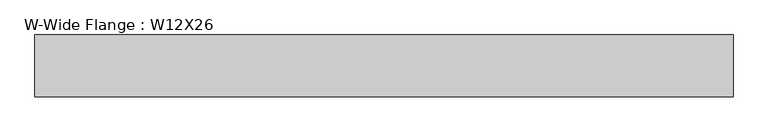
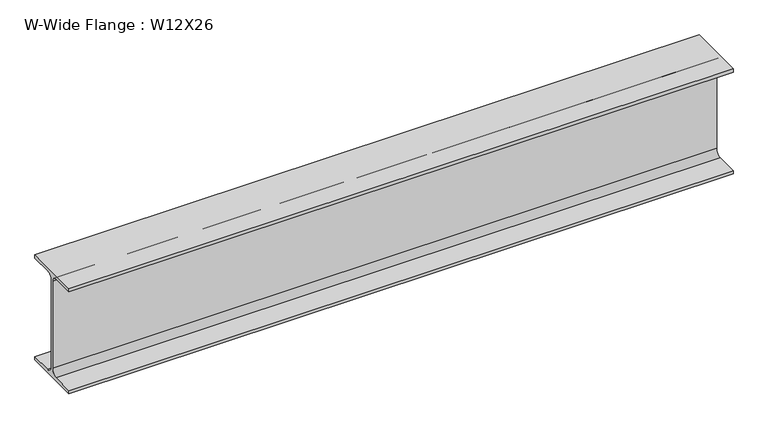
"""IFC4 building model written with IfcOpenShell, lengths in millimetres: beam geometry, W-Wide Flange : W12X26."""

from ifc_helpers import new_model, si_unit, point, frame, frame_2d, origin, place, context, project, spatial, polyline, circle_curve, trimmed, segment, composite_curve, outline, extrude, source, transform, mapped, element, save


def w_wide_flange_w12x26_3993bfbb(model_context):
    return source(origin(), model_context, "Body", "SweptSolid", [
        extrude(outline(composite_curve([segment(polyline([(-82.4011719, -145.5539063), (-20.2902344, -145.5539063)]), True, "CONTINUOUS"), segment(trimmed(circle_curve(frame_2d((-20.2902344, -128.190625)), 17.3632812), [point((-20.2902344, -145.5539063))], [point((-2.9269531, -128.190625))], True, "CARTESIAN"), True, "CONTINUOUS"), segment(polyline([(-2.9269531, -128.190625), (-2.9269531, 128.190625)]), True, "CONTINUOUS"), segment(trimmed(circle_curve(frame_2d((-20.2902344, 128.190625)), 17.3632812), [point((-2.9269531, 128.190625))], [point((-20.2902344, 145.5539062))], True, "CARTESIAN"), True, "CONTINUOUS"), segment(polyline([(-20.2902344, 145.5539062), (-82.4011719, 145.5539062), (-82.4011719, 155.178125), (82.4011719, 155.178125), (82.4011719, 145.5539062), (20.2902344, 145.5539062)]), True, "CONTINUOUS"), segment(trimmed(circle_curve(frame_2d((20.2902344, 128.190625)), 17.3632812), [point((20.2902344, 145.5539062))], [point((2.9269531, 128.190625))], True, "CARTESIAN"), True, "CONTINUOUS"), segment(polyline([(2.9269531, 128.190625), (2.9269531, -128.190625)]), True, "CONTINUOUS"), segment(trimmed(circle_curve(frame_2d((20.2902344, -128.190625)), 17.3632812), [point((2.9269531, -128.190625))], [point((20.2902344, -145.5539063))], True, "CARTESIAN"), True, "CONTINUOUS"), segment(polyline([(20.2902344, -145.5539063), (82.4011719, -145.5539063), (82.4011719, -155.178125), (-82.4011719, -155.178125), (-82.4011719, -145.5539063)]), True, "CONTINUOUS")], self_intersect=False)), frame((-877.2009341, 0.0, 0.0), z_axis=(1.0, 0.0, 0.0), x_axis=(0.0, 1.0, 0.0)), (0.0, 0.0, 1.0), 1855.1009341),
    ])


if __name__ == "__main__":
    model = new_model("IFC4")
    model_context = context("Model", 3, world=origin())
    ifc_project = project(units=[si_unit("LENGTHUNIT", "METRE", prefix="MILLI")], contexts=[model_context])
    site = spatial("IfcSite", under=ifc_project)
    building = spatial("IfcBuilding", under=site)
    placement = place(None, origin())
    w_wide_flange_w12x26_shape = w_wide_flange_w12x26_3993bfbb(model_context)
    element("IfcBeam", 1, ObjectType="W-Wide Flange : W12X26", at=placement, inside=building, context=model_context, shape_type="MappedRepresentation", body=[
        mapped(w_wide_flange_w12x26_shape, transform((0.0, 0.0, 0.0), x_axis=(1.0, 0.0, 0.0), y_axis=(0.0, 1.0, 0.0), z_axis=(0.0, 0.0, 1.0))),
    ])
    save(model, "model.ifc")

# Revit data of these elements
# Type "W-Wide Flange : W12X26"
#   Assembly Code = "B10"
#   W = 26
#   Start Extension Calculation [instance default] = 10' - 0"
#   Start Extension [instance default] = -0' - 0 1/2"
#   End Extension Calculation [instance default] = 10' - 0"
#   End Extension [instance default] = -0' - 0 1/2"
#   Length [instance default] = 5' - 0"
#   bf = 0' - 6 125/256"
#   d = 1' - 0 7/32"
#   k = 0' - 1 1/16"
#   k2 = 0' - 0 175/256"
#   tf = 0' - 0 97/256"
#   tw = 0' - 0 59/256"
#   A = 0.05 SF
#   Beam Material [instance default] = Metal - Steel - ASTM A992
# Element 1 (IfcBeam, "W-Wide Flange : W12X26")
#   Start Extension Calculation = 9' - 1.78547"
#   Start Extension = -0' - 10.71453"
#   Materials on its faces: "Metal - Steel - ASTM A992"
# Materials
#   "Metal - Steel - ASTM A992": class "Metal", colour RGB 128 0 0, transparency 0
